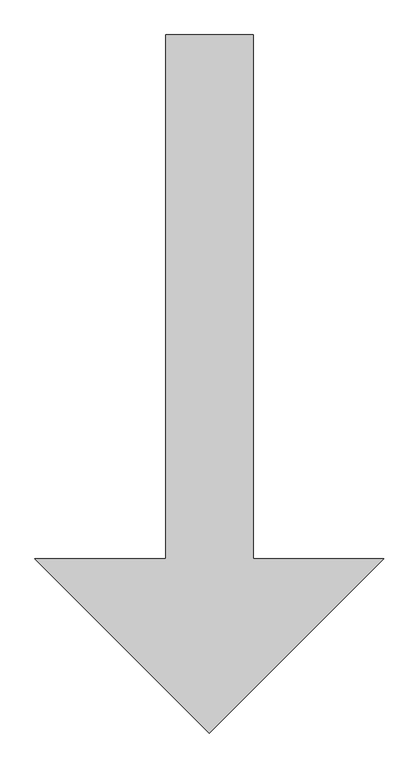
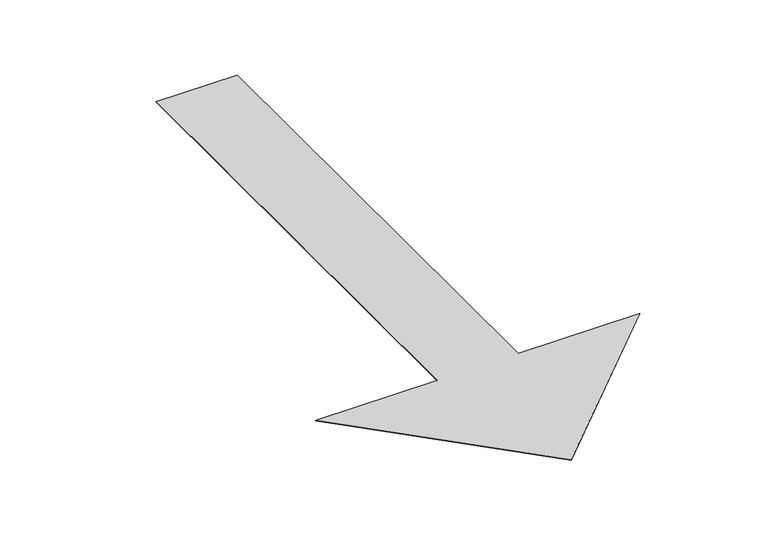
"""IFC4 building model written with IfcOpenShell, lengths in millimetres: proxy geometry, NLRS_90_PA_LB_pijl bewegwijzering_gen_rsf : pijl bewegwijzering."""

from ifc_helpers import new_model, si_unit, origin, origin_with_axes, place, context, project, spatial, polyline, outline, extrude, source, transform, mapped, element, save


def parking_90e2ee20(model_context):
    return source(origin(), model_context, "Body", "SweptSolid", [
        extrude(outline(polyline([(-125.0, 0.0), (-625.0, 500.0), (-250.0, 500.0), (-250.0, 2000.0), (0.0, 2000.0), (0.0, 500.0), (375.0, 500.0), (-125.0, 0.0)])), origin_with_axes(), (0.0, 0.0, 1.0), 1.0),
    ])


if __name__ == "__main__":
    model = new_model("IFC4")
    model_context = context("Model", 3, world=origin())
    ifc_project = project(units=[si_unit("LENGTHUNIT", "METRE", prefix="MILLI")], contexts=[model_context])
    site = spatial("IfcSite", under=ifc_project)
    building = spatial("IfcBuilding", under=site)
    placement = place(None, origin())
    parking_shape = parking_90e2ee20(model_context)
    element("IfcBuildingElementProxy", 1, Name="NLRS_90_PA_LB_pijl bewegwijzering_gen_rsf : pijl bewegwijzering", ObjectType="NLRS_90_PA_LB_pijl bewegwijzering_gen_rsf : pijl bewegwijzering", at=placement, inside=building, context=model_context, shape_type="MappedRepresentation", body=[
        mapped(parking_shape, transform((0.0, 0.0, 0.0), x_axis=(1.0, 0.0, 0.0), y_axis=(0.0, 1.0, 0.0), z_axis=(0.0, 0.0, 1.0))),
    ])
    save(model, "model.ifc")

# Revit data of these elements
# Type "NLRS_90_PA_LB_pijl bewegwijzering_gen_rsf : pijl bewegwijzering"
#   Type IFC Predefined Type = "USERDEFINED"
#   Export Type to IFC As = "IfcBuildingElementProxyType"
#   Type IfcGUID = "2C9lkgojj1sel6c4s_vQ2Q"
#   IfcName[Type] = "pijl bewegwijzering"
#   IfcDescription[Type] = "pijl bewegwijzering"
#   IfcObjectType[Type] = "SIGNAGE"
#   IfcExportAs[Type] = "IfcBuildingElementProxyType"
#   IfcExportType[Type] = "USERDEFINED"
#   Description = "pijl bewegwijzering"
#   Assembly Code = "90.72"
#   Pijlbreedte = 250.00 mm
#   Lengte_pijl = 2000.00 mm
#   Dikte_belijning = 1.00 mm
#   Materiaal_belijning = NLRS_v4_verf ivoorkleurig mat_gen_rsf
# Element 1 (IfcBuildingElementProxy, "NLRS_90_PA_LB_pijl bewegwijzering_gen_rsf : pijl bewegwijzering")
#   Materials on its faces: "NLRS_v4_verf ivoorkleurig mat_gen_rsf"
# Materials
#   "NLRS_v4_verf ivoorkleurig mat_gen_rsf": class "V - Verven", colour RGB 216 216 204, transparency 0, Keynote = "v4", Manufacturer = "Revit Standards Foundation", URL = "www.revitstandards.org", Description = "verf ivoorkleurig mat", Cost = 0
